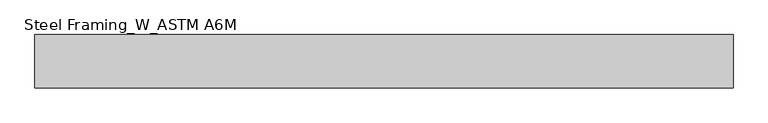
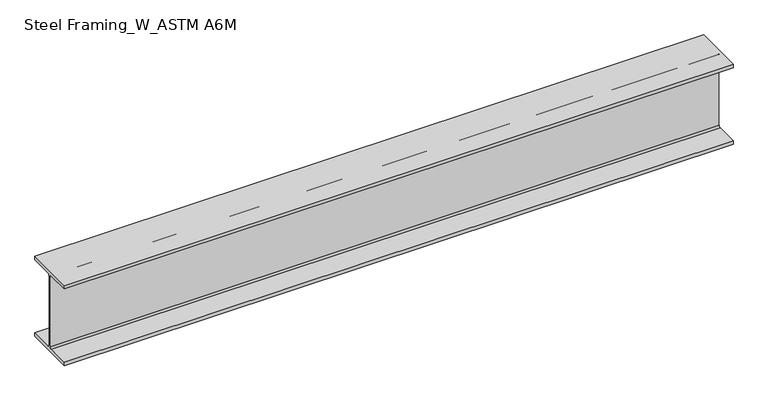
"""IFC4 building model written with IfcOpenShell, lengths in millimetres: beam geometry, Steel Framing_W_ASTM A6M : H_SB_AR_S02_W460x128_B1."""

from ifc_helpers import new_model, si_unit, point, frame, frame_2d, origin, place, context, project, spatial, polyline, circle_curve, trimmed, segment, composite_curve, outline, extrude, source, transform, mapped, element, save


def steel_framing_w_astm_a6m_196e06da(model_context):
    return source(origin(), model_context, "Body", "SweptSolid", [
        extrude(outline(composite_curve([segment(polyline([(141.0, -213.9), (141.0, -233.5), (-141.0, -233.5), (-141.0, -213.9), (-16.2, -213.9)]), True, "CONTINUOUS"), segment(trimmed(circle_curve(frame_2d((-16.2, -203.8)), 10.1), [point((-16.2, -213.9))], [point((-6.1, -203.8))], True, "CARTESIAN"), True, "CONTINUOUS"), segment(polyline([(-6.1, -203.8), (-6.1, 203.8)]), True, "CONTINUOUS"), segment(trimmed(circle_curve(frame_2d((-16.2, 203.8)), 10.1), [point((-6.1, 203.8))], [point((-16.2, 213.9))], True, "CARTESIAN"), True, "CONTINUOUS"), segment(polyline([(-16.2, 213.9), (-141.0, 213.9), (-141.0, 233.5), (141.0, 233.5), (141.0, 213.9), (16.2, 213.9)]), True, "CONTINUOUS"), segment(trimmed(circle_curve(frame_2d((16.2, 203.8)), 10.1), [point((16.2, 213.9))], [point((6.1, 203.8))], True, "CARTESIAN"), True, "CONTINUOUS"), segment(polyline([(6.1, 203.8), (6.1, -203.8)]), True, "CONTINUOUS"), segment(trimmed(circle_curve(frame_2d((16.2, -203.8)), 10.1), [point((6.1, -203.8))], [point((16.2, -213.9))], True, "CARTESIAN"), True, "CONTINUOUS"), segment(polyline([(16.2, -213.9), (141.0, -213.9)]), True, "CONTINUOUS")], self_intersect=False)), frame((-1846.3, 0.0, 0.0), z_axis=(1.0, 0.0, 0.0), x_axis=(0.0, 1.0, 0.0)), (0.0, 0.0, 1.0), 3692.6),
    ])


if __name__ == "__main__":
    model = new_model("IFC4")
    model_context = context("Model", 3, world=origin())
    ifc_project = project(units=[si_unit("LENGTHUNIT", "METRE", prefix="MILLI")], contexts=[model_context])
    site = spatial("IfcSite", under=ifc_project)
    building = spatial("IfcBuilding", under=site)
    placement = place(None, origin())
    steel_framing_w_astm_a6m_shape = steel_framing_w_astm_a6m_196e06da(model_context)
    element("IfcBeam", 1, ObjectType="Steel Framing_W_ASTM A6M : H_SB_AR_S02_W460x128_B1", at=placement, inside=building, context=model_context, shape_type="MappedRepresentation", body=[
        mapped(steel_framing_w_astm_a6m_shape, transform((0.0, 0.0, 0.0), x_axis=(1.0, 0.0, 0.0), y_axis=(0.0, 1.0, 0.0), z_axis=(0.0, 0.0, 1.0))),
    ])
    save(model, "model.ifc")

# Revit data of these elements
# Type "Steel Framing_W_ASTM A6M : H_SB_AR_S02_W460x128_B1"
#   Section Name Key = "W18x86"
#   Width = 28.2 cm
#   Web Thickness = 1.22 cm
#   Web Fillet = 1.01 cm
#   Warping Constant = 3650000.0 cm⁶
#   Torsional Moment of Inertia = 171.00 cm⁴
#   Section Area = 163.0 cm²
#   Plastic Modulus weak axis = 793.0 cm³
#   Plastic Modulus strong axis = 3050.0 cm³
#   Perimeter = 2.02 m²/m
#   Nominal Weight = 128.00 kgf/m
#   Moment of Inertia weak axis = 7280.00 cm⁴
#   Moment of Inertia strong axis = 63700.00 cm⁴
#   Height = 46.7 cm
#   Flange Thickness = 1.96 cm
#   Elastic Modulus weak axis = 518.0 cm³
#   Elastic Modulus strong axis = 2720.0 cm³
#   Centroid Vertical = 23.35 cm
#   Centroid Horizontal = 14.1 cm
#   Length [instance default] = 1500 mm
#   Structural Material [instance default] = Steel, 45-345
#   Bolt Spacing = 0
#   Assembly Code = ""
# Element 1 (IfcBeam, "Steel Framing_W_ASTM A6M : H_SB_AR_S02_W460x128_B1")
#   Materials on its faces: "Steel, 45-345"
# Materials
#   "Steel, 45-345": class "Metal", colour RGB 189 187 185, transparency 0, Description = "Steel 345 MPa", Cost = 0
